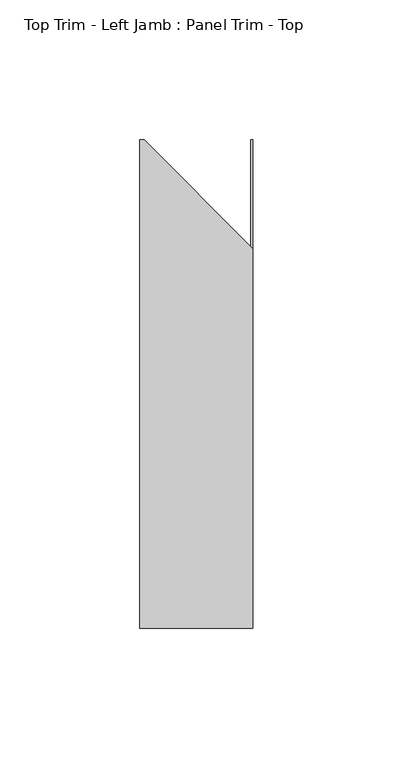
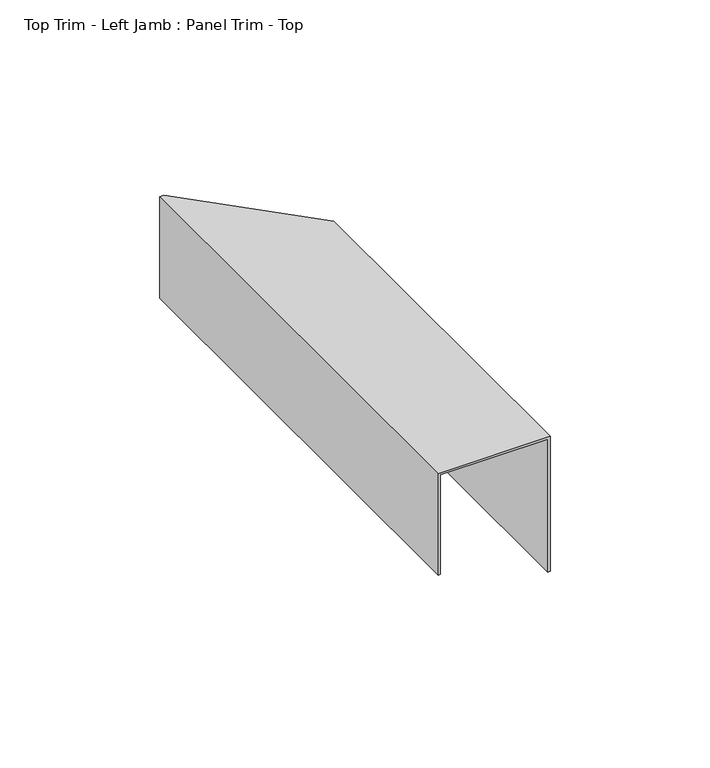
"""IFC4 building model written with IfcOpenShell, lengths in millimetres: proxy geometry, Top Trim - Left Jamb : Panel Trim - Top."""

from ifc_helpers import new_model, si_unit, origin, place, context, project, spatial, faceted_brep, source, transform, mapped, element, save


def top_trim_left_jamb_panel_trim_top_cc1ac03c(model_context):
    return source(origin(), model_context, "Body", "Brep", [
        faceted_brep([(587327.0060739, -531601.1163841, 2439.9875), (587327.0060739, -531601.1163841, 2401.8875), (587326.2186739, -531601.1163841, 2401.8875), (587326.2186739, -531601.1163841, 2440.78125), (587327.7847411, -531601.1163841, 2440.78125), (587327.7847411, -531601.1163841, 2439.9875), (587366.6808739, -531601.1163841, 2389.1875), (587365.8934739, -531601.1163841, 2389.1875), (587365.8934739, -531601.1163841, 2413.0), (587366.6808739, -531601.1163841, 2413.0), (587327.0060739, -531775.7413841, 2439.9875), (587365.8934739, -531775.7413841, 2439.9875), (587365.8934739, -531775.7413841, 2389.1875), (587366.6808739, -531775.7413841, 2389.1875), (587366.6808739, -531775.7413841, 2440.78125), (587326.2186739, -531775.7413841, 2440.78125), (587326.2186739, -531775.7413841, 2401.8875), (587327.0060739, -531775.7413841, 2401.8875), (587366.6808739, -531640.0125169, 2440.78125), (587366.6808739, -531640.0125169, 2413.0), (587365.8934739, -531639.2251169, 2439.9875), (587365.8934739, -531639.2251169, 2413.0)], [[[0, 1, 2, 3, 4, 5]], [[6, 7, 8, 9]], [[10, 11, 12, 13, 14, 15, 16, 17]], [[1, 0, 10, 17]], [[2, 1, 17, 16]], [[3, 2, 16, 15]], [[15, 14, 18, 4, 3]], [[14, 13, 6, 9, 19, 18]], [[7, 6, 13, 12]], [[12, 11, 20, 21, 8, 7]], [[11, 10, 0, 5, 20]], [[21, 19, 9, 8]], [[19, 21, 20, 5, 4, 18]]]),
    ])


if __name__ == "__main__":
    model = new_model("IFC4")
    model_context = context("Model", 3, world=origin())
    ifc_project = project(units=[si_unit("LENGTHUNIT", "METRE", prefix="MILLI")], contexts=[model_context])
    site = spatial("IfcSite", under=ifc_project)
    building = spatial("IfcBuilding", under=site)
    placement = place(None, origin())
    top_trim_left_jamb_panel_trim_top_shape = top_trim_left_jamb_panel_trim_top_cc1ac03c(model_context)
    element("IfcBuildingElementProxy", 1, Name="Top Trim - Left Jamb : Panel Trim - Top", ObjectType="Top Trim - Left Jamb : Panel Trim - Top", at=placement, inside=building, context=model_context, shape_type="MappedRepresentation", body=[
        mapped(top_trim_left_jamb_panel_trim_top_shape, transform((0.0, 0.0, 0.0), x_axis=(1.0, 0.0, 0.0), y_axis=(0.0, 1.0, 0.0), z_axis=(0.0, 0.0, 1.0))),
    ])
    save(model, "model.ifc")

# Revit data of these elements
# Element 1 (IfcBuildingElementProxy, "Top Trim - Left Jamb : Panel Trim - Top")
#   Materials on its faces: "EDGE TRIM BY MTL PANEL MFR."
# Materials
#   "EDGE TRIM BY MTL PANEL MFR.": class "Generic", colour RGB 239 242 240, transparency 0, Cost = 0
